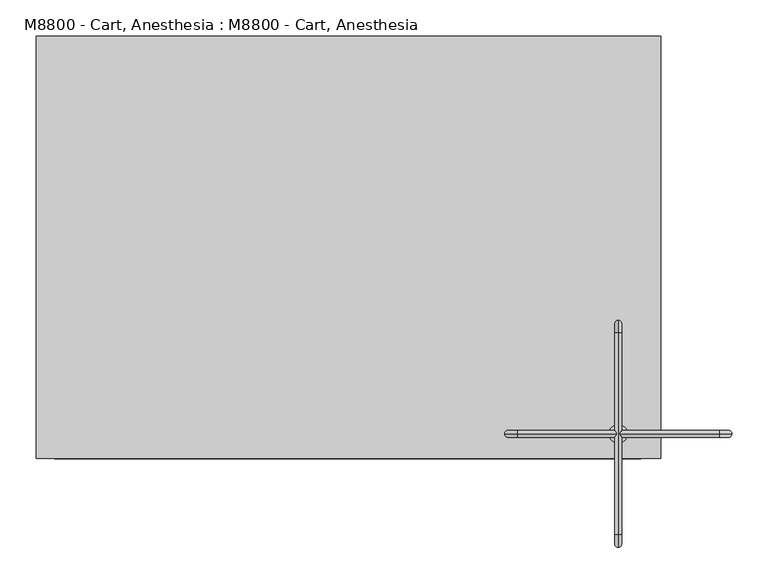
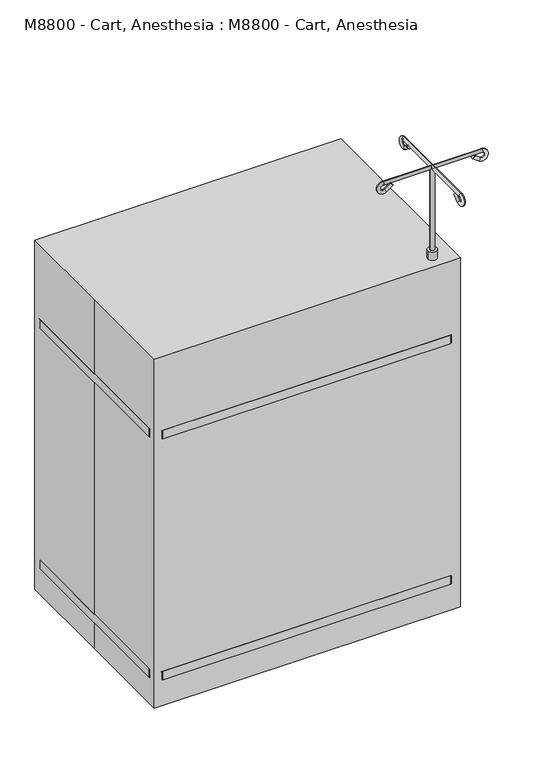
"""IFC4 building model written with IfcOpenShell, lengths in millimetres: proxy geometry, M8800 - Cart, Anesthesia : M8800 - Cart, Anesthesia."""

from ifc_helpers import new_model, si_unit, point, frame, frame_2d, origin, origin_with_axes, place, context, project, spatial, polyline, circle_curve, ellipse_curve, trimmed, segment, composite_curve, outline, extrude, source, transform, mapped, element, save
from ifc_brep_helpers import plane_surface, cylinder_surface, revolved_surface, advanced_brep


def m8800_cart_anesthesia_m8800_cart_anesthesia_5f1830e2(model_context):
    return source(origin(), model_context, "Body", "SolidModel", [
        extrude(outline(composite_curve([segment(trimmed(circle_curve(frame_2d((372.8549743, -257.8577972)), 6.35), [point((366.5049743, -257.8577972))], [point((379.2049743, -257.8577972))], False, "CARTESIAN"), True, "CONTINUOUS"), segment(trimmed(circle_curve(frame_2d((372.8549743, -257.8577972)), 6.35), [point((379.2049743, -257.8577972))], [point((366.5049743, -257.8577972))], False, "CARTESIAN"), True, "CONTINUOUS")], self_intersect=False)), frame((0.0, 0.0, 1066.8), z_axis=(0.0, 0.0, 1.0), x_axis=(1.0, 0.0, 0.0)), (0.0, 0.0, 1.0), 247.65),
        advanced_brep(
        [(372.8549743, -375.3332189, 1305.9580135), (372.8549743, -369.7574508, 1298.2355504), (372.8549743, -387.3355558, 1285.5438178), (372.8549743, -392.9113238, 1293.2662808), (372.8549743, -397.5577972, 1317.1641667), (372.8549743, -397.5577972, 1307.6391667), (372.8549743, -118.1577972, 1317.1641667), (372.8549743, -118.1577972, 1307.6391667), (372.8549743, -128.3800387, 1285.5438178), (372.8549743, -122.8042706, 1293.2662808), (372.8549743, -140.3823755, 1305.9580135), (372.8549743, -145.9581436, 1298.2355504)],
        [
            (0, 1, circle_curve(frame((372.8549743, -372.5453349, 1302.096782), z_axis=(0.0, 0.8107572744902805, 0.5853824748496425), x_axis=(0.0, 0.5853824748496425, -0.8107572744902805)), 4.7625)),
            (1, 0, circle_curve(frame((372.8549743, -372.5453349, 1302.096782), z_axis=(0.0, 0.8107572744902805, 0.5853824748496425), x_axis=(0.0, 0.5853824748496425, -0.8107572744902805)), 4.7625)),
            (1, 2),
            (2, 3, circle_curve(frame((372.8549743, -390.1234398, 1289.4050493), z_axis=(0.0, 0.8107572744902805, 0.5853824748496425), x_axis=(0.0, 0.5853824748496425, -0.8107572744902805)), 4.7625)),
            (3, 0),
            (3, 2, circle_curve(frame((372.8549743, -390.1234398, 1289.4050493), z_axis=(0.0, 0.8107572744902805, 0.5853824748496425), x_axis=(0.0, 0.5853824748496425, -0.8107572744902805)), 4.7625)),
            (4, 5, circle_curve(frame((372.8549743, -397.5577972, 1312.4016667), z_axis=(0.0, -1.0, 0.0), x_axis=(0.0, 0.0, 1.0)), 4.7625)),
            (5, 3, circle_curve(frame((372.8549743, -397.5577972, 1299.7016667), z_axis=(1.0, 0.0, 0.0), x_axis=(0.0, 0.5853824748496496, -0.8107572744902752)), 7.9375)),
            (2, 4, circle_curve(frame((372.8549743, -397.5577972, 1299.7016667), z_axis=(-1.0, 0.0, 0.0), x_axis=(0.0, 0.5853824748496496, -0.8107572744902752)), 17.4625)),
            (5, 4, circle_curve(frame((372.8549743, -397.5577972, 1312.4016667), z_axis=(0.0, -1.0, 0.0), x_axis=(0.0, 0.0, 1.0)), 4.7625)),
            (4, 6),
            (6, 7, circle_curve(frame((372.8549743, -118.1577972, 1312.4016667), z_axis=(0.0, -1.0, 0.0), x_axis=(0.0, 0.0, 1.0)), 4.7625)),
            (7, 5),
            (7, 6, circle_curve(frame((372.8549743, -118.1577972, 1312.4016667), z_axis=(0.0, -1.0, 0.0), x_axis=(0.0, 0.0, 1.0)), 4.7625)),
            (8, 9, circle_curve(frame((372.8549743, -125.5921547, 1289.4050493), z_axis=(0.0, 0.8107572744895717, -0.5853824748506239), x_axis=(0.0, -0.5853824748506239, -0.8107572744895717)), 4.7625)),
            (9, 7, circle_curve(frame((372.8549743, -118.1577972, 1299.7016667), z_axis=(1.0, 0.0, 0.0), x_axis=(0.0, 0.0, 1.0)), 7.9375)),
            (6, 8, circle_curve(frame((372.8549743, -118.1577972, 1299.7016667), z_axis=(-1.0, 0.0, 0.0), x_axis=(0.0, 0.0, 1.0)), 17.4625)),
            (9, 8, circle_curve(frame((372.8549743, -125.5921547, 1289.4050493), z_axis=(0.0, 0.8107572744906105, -0.585382474849185), x_axis=(0.0, -0.585382474849185, -0.8107572744906105)), 4.7625)),
            (10, 11, circle_curve(frame((372.8549743, -143.1702596, 1302.096782), z_axis=(0.0, -0.8107572744898957, 0.5853824748501752), x_axis=(0.0, -0.5853824748501752, -0.8107572744898957)), 4.7625)),
            (11, 10, circle_curve(frame((372.8549743, -143.1702596, 1302.096782), z_axis=(0.0, -0.8107572744898957, 0.5853824748501752), x_axis=(0.0, -0.5853824748501752, -0.8107572744898957)), 4.7625)),
            (8, 11),
            (10, 9),
        ],
        [
            plane_surface(frame((639.5549743, -372.5453349, 1302.096782), z_axis=(0.0, 0.8107572744902805, 0.5853824748496425), x_axis=(-1.0, 0.0, 0.0))),
            cylinder_surface(frame((372.8549743, -372.5453349, 1302.096782), z_axis=(0.0, 0.8107572744902805, 0.5853824748496425), x_axis=(0.0, 0.5853824748496425, -0.8107572744902805)), 4.7625),
            revolved_surface(trimmed(ellipse_curve(frame((372.8549743, -390.1234398, 1289.4050493), z_axis=(0.0, -0.8107572744902751, -0.5853824748496497), x_axis=(0.0, 0.5853824748496497, -0.8107572744902751)), 4.7625, 4.7625), [point((372.8549743, -392.9113238, 1293.2662808))], [point((372.8549743, -387.3355558, 1285.5438178))], True, "CARTESIAN"), (639.5549743, -397.5577972, 1299.7016667), (1.0, 0.0, 0.0)),
            revolved_surface(trimmed(ellipse_curve(frame((372.8549743, -390.1234398, 1289.4050493), z_axis=(0.0, -0.8107572744902751, -0.5853824748496497), x_axis=(0.0, 0.5853824748496497, -0.8107572744902751)), 4.7625, 4.7625), [point((372.8549743, -387.3355558, 1285.5438178))], [point((372.8549743, -392.9113238, 1293.2662808))], True, "CARTESIAN"), (639.5549743, -397.5577972, 1299.7016667), (1.0, 0.0, 0.0)),
            cylinder_surface(frame((372.8549743, -397.5577972, 1312.4016667), z_axis=(0.0, -1.0, 0.0), x_axis=(0.0, 0.0, 1.0)), 4.7625),
            revolved_surface(trimmed(ellipse_curve(frame((372.8549743, -118.1577972, 1312.4016667), z_axis=(0.0, 1.0, 0.0), x_axis=(0.0, 0.0, 1.0)), 4.7625, 4.7625), [point((372.8549743, -118.1577972, 1307.6391667))], [point((372.8549743, -118.1577972, 1317.1641667))], True, "CARTESIAN"), (639.5549743, -118.1577972, 1299.7016667), (1.0, 0.0, 0.0)),
            revolved_surface(trimmed(ellipse_curve(frame((372.8549743, -118.1577972, 1312.4016667), z_axis=(0.0, 1.0, 0.0), x_axis=(0.0, 0.0, 1.0)), 4.7625, 4.7625), [point((372.8549743, -118.1577972, 1317.1641667))], [point((372.8549743, -118.1577972, 1307.6391667))], True, "CARTESIAN"), (639.5549743, -118.1577972, 1299.7016667), (1.0, 0.0, 0.0)),
            plane_surface(frame((639.5549743, -143.1702596, 1302.096782), z_axis=(0.0, -0.8107572744898955, 0.5853824748501754), x_axis=(-1.0, 0.0, 0.0))),
            cylinder_surface(frame((372.8549743, -125.5921547, 1289.4050493), z_axis=(0.0, 0.8107572744898957, -0.5853824748501752), x_axis=(0.0, -0.5853824748501752, -0.8107572744898957)), 4.7625),
        ],
        [
            (0, [[1, 2]]),
            (1, [[3, 4, 5, -2]]),
            (1, [[-5, 6, -3, -1]]),
            (2, [[7, 8, -4, 9]]),
            (3, [[10, -9, -6, -8]]),
            (4, [[11, 12, 13, -7]]),
            (4, [[-13, 14, -11, -10]]),
            (5, [[15, 16, -12, 17]]),
            (6, [[18, -17, -14, -16]]),
            (7, [[19, 20]]),
            (8, [[21, -19, 22, -15]]),
            (8, [[-22, -20, -21, -18]]),
        ],
    ),
        advanced_brep(
        [(255.3795526, -257.8577972, 1305.9580135), (260.9553207, -257.8577972, 1298.2355504), (243.3772158, -257.8577972, 1285.5438178), (237.8014477, -257.8577972, 1293.2662808), (233.1549743, -257.8577972, 1317.1641667), (233.1549743, -257.8577972, 1307.6391667), (512.5549743, -257.8577972, 1317.1641667), (512.5549743, -257.8577972, 1307.6391667), (502.3327328, -257.8577972, 1285.5438178), (507.9085009, -257.8577972, 1293.2662808), (490.330396, -257.8577972, 1305.9580135), (484.7546279, -257.8577972, 1298.2355504)],
        [
            (0, 1, circle_curve(frame((258.1674367, -257.8577972, 1302.096782), z_axis=(0.810757274490287, 0.0, 0.5853824748496332), x_axis=(0.5853824748496332, 0.0, -0.810757274490287)), 4.7625)),
            (1, 0, circle_curve(frame((258.1674367, -257.8577972, 1302.096782), z_axis=(0.810757274490287, 0.0, 0.5853824748496332), x_axis=(0.5853824748496332, 0.0, -0.810757274490287)), 4.7625)),
            (1, 2),
            (2, 3, circle_curve(frame((240.5893317, -257.8577972, 1289.4050493), z_axis=(0.810757274490287, 0.0, 0.5853824748496332), x_axis=(0.5853824748496332, 0.0, -0.810757274490287)), 4.7625)),
            (3, 0),
            (3, 2, circle_curve(frame((240.5893317, -257.8577972, 1289.4050493), z_axis=(0.810757274490287, 0.0, 0.5853824748496332), x_axis=(0.5853824748496332, 0.0, -0.810757274490287)), 4.7625)),
            (4, 5, circle_curve(frame((233.1549743, -257.8577972, 1312.4016667), z_axis=(-1.0, 0.0, 0.0), x_axis=(0.0, 0.0, 1.0)), 4.7625)),
            (5, 3, circle_curve(frame((233.1549743, -257.8577972, 1299.7016667), z_axis=(0.0, -1.0, 0.0), x_axis=(0.5853824748496301, 0.0, -0.8107572744902892)), 7.9375)),
            (2, 4, circle_curve(frame((233.1549743, -257.8577972, 1299.7016667), z_axis=(0.0, 1.0, 0.0), x_axis=(0.5853824748496301, 0.0, -0.8107572744902892)), 17.4625)),
            (5, 4, circle_curve(frame((233.1549743, -257.8577972, 1312.4016667), z_axis=(-1.0, 0.0, 0.0), x_axis=(0.0, 0.0, 1.0)), 4.7625)),
            (4, 6),
            (6, 7, circle_curve(frame((512.5549743, -257.8577972, 1312.4016667), z_axis=(-1.0, 0.0, 0.0), x_axis=(0.0, 0.0, 1.0)), 4.7625)),
            (7, 5),
            (7, 6, circle_curve(frame((512.5549743, -257.8577972, 1312.4016667), z_axis=(-1.0, 0.0, 0.0), x_axis=(0.0, 0.0, 1.0)), 4.7625)),
            (8, 9, circle_curve(frame((505.1206169, -257.8577972, 1289.4050493), z_axis=(0.8107572744899113, 0.0, -0.5853824748501535), x_axis=(-0.5853824748501535, 0.0, -0.8107572744899113)), 4.7625)),
            (9, 7, circle_curve(frame((512.5549743, -257.8577972, 1299.7016667), z_axis=(0.0, -1.0, 0.0), x_axis=(0.0, 0.0, 1.0)), 7.9375)),
            (6, 8, circle_curve(frame((512.5549743, -257.8577972, 1299.7016667), z_axis=(0.0, 1.0, 0.0), x_axis=(0.0, 0.0, 1.0)), 17.4625)),
            (9, 8, circle_curve(frame((505.1206169, -257.8577972, 1289.4050493), z_axis=(0.8107572744899163, 0.0, -0.5853824748501466), x_axis=(-0.5853824748501466, 0.0, -0.8107572744899163)), 4.7625)),
            (10, 11, circle_curve(frame((487.5425119, -257.8577972, 1302.096782), z_axis=(-0.8107572744899004, 0.0, 0.5853824748501685), x_axis=(-0.5853824748501685, 0.0, -0.8107572744899004)), 4.7625)),
            (11, 10, circle_curve(frame((487.5425119, -257.8577972, 1302.096782), z_axis=(-0.8107572744899004, 0.0, 0.5853824748501685), x_axis=(-0.5853824748501685, 0.0, -0.8107572744899004)), 4.7625)),
            (8, 11),
            (10, 9),
        ],
        [
            plane_surface(frame((258.1674367, -473.7577972, 1302.096782), z_axis=(0.810757274490287, 0.0, 0.5853824748496332), x_axis=(0.0, 1.0, 0.0))),
            cylinder_surface(frame((258.1674367, -257.8577972, 1302.096782), z_axis=(0.810757274490287, 0.0, 0.5853824748496332), x_axis=(0.5853824748496332, 0.0, -0.810757274490287)), 4.7625),
            revolved_surface(trimmed(ellipse_curve(frame((240.5893317, -257.8577972, 1289.4050493), z_axis=(-0.8107572744902892, 0.0, -0.5853824748496301), x_axis=(0.5853824748496301, 0.0, -0.8107572744902892)), 4.7625, 4.7625), [point((237.8014477, -257.8577972, 1293.2662808))], [point((243.3772158, -257.8577972, 1285.5438178))], True, "CARTESIAN"), (233.1549743, -473.7577972, 1299.7016667), (0.0, -1.0, 0.0)),
            revolved_surface(trimmed(ellipse_curve(frame((240.5893317, -257.8577972, 1289.4050493), z_axis=(-0.8107572744902892, 0.0, -0.5853824748496301), x_axis=(0.5853824748496301, 0.0, -0.8107572744902892)), 4.7625, 4.7625), [point((243.3772158, -257.8577972, 1285.5438178))], [point((237.8014477, -257.8577972, 1293.2662808))], True, "CARTESIAN"), (233.1549743, -473.7577972, 1299.7016667), (0.0, -1.0, 0.0)),
            cylinder_surface(frame((233.1549743, -257.8577972, 1312.4016667), z_axis=(-1.0, 0.0, 0.0), x_axis=(0.0, 0.0, 1.0)), 4.7625),
            revolved_surface(trimmed(ellipse_curve(frame((512.5549743, -257.8577972, 1312.4016667), z_axis=(1.0, 0.0, 0.0), x_axis=(0.0, 0.0, 1.0)), 4.7625, 4.7625), [point((512.5549743, -257.8577972, 1307.6391667))], [point((512.5549743, -257.8577972, 1317.1641667))], True, "CARTESIAN"), (512.5549743, -473.7577972, 1299.7016667), (0.0, -1.0, 0.0)),
            revolved_surface(trimmed(ellipse_curve(frame((512.5549743, -257.8577972, 1312.4016667), z_axis=(1.0, 0.0, 0.0), x_axis=(0.0, 0.0, 1.0)), 4.7625, 4.7625), [point((512.5549743, -257.8577972, 1317.1641667))], [point((512.5549743, -257.8577972, 1307.6391667))], True, "CARTESIAN"), (512.5549743, -473.7577972, 1299.7016667), (0.0, -1.0, 0.0)),
            plane_surface(frame((487.5425119, -473.7577972, 1302.096782), z_axis=(-0.8107572744899004, 0.0, 0.5853824748501685), x_axis=(0.0, 1.0, 0.0))),
            cylinder_surface(frame((505.1206169, -257.8577972, 1289.4050493), z_axis=(0.8107572744899004, 0.0, -0.5853824748501685), x_axis=(-0.5853824748501685, 0.0, -0.8107572744899004)), 4.7625),
        ],
        [
            (0, [[1, 2]]),
            (1, [[3, 4, 5, -2]]),
            (1, [[-5, 6, -3, -1]]),
            (2, [[7, 8, -4, 9]]),
            (3, [[10, -9, -6, -8]]),
            (4, [[11, 12, 13, -7]]),
            (4, [[-13, 14, -11, -10]]),
            (5, [[15, 16, -12, 17]]),
            (6, [[18, -17, -14, -16]]),
            (7, [[19, 20]]),
            (8, [[21, -19, 22, -15]]),
            (8, [[-22, -20, -21, -18]]),
        ],
    ),
        extrude(outline(polyline([(820.0646026, -374.65), (966.1146026, -374.65), (966.1146026, 120.65), (820.0646026, 120.65), (820.0646026, 127.0), (972.4646026, 127.0), (972.4646026, -381.0), (820.0646026, -381.0), (820.0646026, -374.65)])), frame((0.0, -257.8577972, 0.0), z_axis=(0.0, 1.0, 0.0), x_axis=(0.0, 0.0, 1.0)), (0.0, 0.0, 1.0), 25.4),
        extrude(outline(composite_curve([segment(polyline([(404.3351605, -292.1), (-406.4, -292.1)]), True, "CONTINUOUS"), segment(trimmed(circle_curve(frame_2d((-406.4, -266.7)), 25.4), [point((-406.4, -292.1))], [point((-431.8, -266.7))], False, "CARTESIAN"), True, "CONTINUOUS"), segment(polyline([(-431.8, -266.7), (-431.8, 266.9423102)]), True, "CONTINUOUS"), segment(trimmed(circle_curve(frame_2d((-406.4, 266.9423102)), 25.4), [point((-431.8, 266.9423102))], [point((-406.4, 292.3423102))], False, "CARTESIAN"), True, "CONTINUOUS"), segment(polyline([(-406.4, 292.3423102), (404.3351605, 292.3423102)]), True, "CONTINUOUS"), segment(trimmed(circle_curve(frame_2d((404.3351605, 266.9423102)), 25.4), [point((404.3351605, 292.3423102))], [point((429.7351605, 266.9423102))], False, "CARTESIAN"), True, "CONTINUOUS"), segment(polyline([(429.7351605, 266.9423102), (429.7351605, -266.7)]), True, "CONTINUOUS"), segment(trimmed(circle_curve(frame_2d((404.3351605, -266.7)), 25.4), [point((429.7351605, -266.7))], [point((404.3351605, -292.1))], False, "CARTESIAN"), True, "CONTINUOUS")], self_intersect=False)), frame((0.0, 0.0, 794.6646026), z_axis=(0.0, 0.0, 1.0), x_axis=(1.0, 0.0, 0.0)), (0.0, 0.0, 1.0), 25.4),
        extrude(outline(polyline([(-387.35, -260.35), (-387.35, -241.3), (387.35, -241.3), (387.35, -260.35), (-387.35, -260.35)])), frame((0.0, 0.0, 101.6), z_axis=(0.0, 0.0, 1.0), x_axis=(1.0, 0.0, 0.0)), (0.0, 0.0, 1.0), 693.0646026),
        extrude(outline(polyline([(406.4, -260.35), (387.35, -260.35), (387.35, 247.65), (406.4, 247.65), (406.4, -260.35)])), frame((0.0, 0.0, 101.6), z_axis=(0.0, 0.0, 1.0), x_axis=(1.0, 0.0, 0.0)), (0.0, 0.0, 1.0), 693.0646026),
        extrude(outline(polyline([(-387.35, -260.35), (-406.4, -260.35), (-406.4, 247.65), (-387.35, 247.65), (-387.35, -260.35)])), frame((0.0, 0.0, 101.6), z_axis=(0.0, 0.0, 1.0), x_axis=(1.0, 0.0, 0.0)), (0.0, 0.0, 1.0), 693.0646026),
        extrude(outline(polyline([(-228.6, 31.75), (-236.4377343, 76.2), (-208.0622657, 76.2), (-215.9, 31.75), (-228.6, 31.75)])), frame((-374.65, 0.0, 0.0), z_axis=(1.0, 0.0, 0.0), x_axis=(0.0, 1.0, 0.0)), (0.0, 0.0, 1.0), 3.175),
        extrude(outline(polyline([(-228.6, 31.75), (-236.4377343, 76.2), (-208.0622657, 76.2), (-215.9, 31.75), (-228.6, 31.75)])), frame((-390.525, 0.0, 0.0), z_axis=(1.0, 0.0, 0.0), x_axis=(0.0, 1.0, 0.0)), (0.0, 0.0, 1.0), 3.175),
        extrude(outline(composite_curve([segment(trimmed(circle_curve(frame_2d((-222.25, 31.75)), 31.75), [point((-254.0, 31.75))], [point((-190.5, 31.75))], False, "CARTESIAN"), True, "CONTINUOUS"), segment(trimmed(circle_curve(frame_2d((-222.25, 31.75)), 31.75), [point((-190.5, 31.75))], [point((-254.0, 31.75))], False, "CARTESIAN"), True, "CONTINUOUS")], self_intersect=False)), frame((-387.35, 0.0, 0.0), z_axis=(1.0, 0.0, 0.0), x_axis=(0.0, 1.0, 0.0)), (0.0, 0.0, 1.0), 12.7),
        extrude(outline(polyline([(-228.6, 31.75), (-236.4377343, 76.2), (-208.0622657, 76.2), (-215.9, 31.75), (-228.6, 31.75)])), frame((365.125, 0.0, 0.0), z_axis=(1.0, 0.0, 0.0), x_axis=(0.0, 1.0, 0.0)), (0.0, 0.0, 1.0), 3.175),
        extrude(outline(polyline([(-228.6, 31.75), (-236.4377343, 76.2), (-208.0622657, 76.2), (-215.9, 31.75), (-228.6, 31.75)])), frame((381.0, 0.0, 0.0), z_axis=(1.0, 0.0, 0.0), x_axis=(0.0, 1.0, 0.0)), (0.0, 0.0, 1.0), 3.175),
        extrude(outline(composite_curve([segment(trimmed(circle_curve(frame_2d((-222.25, 31.75)), 31.75), [point((-254.0, 31.75))], [point((-190.5, 31.75))], False, "CARTESIAN"), True, "CONTINUOUS"), segment(trimmed(circle_curve(frame_2d((-222.25, 31.75)), 31.75), [point((-190.5, 31.75))], [point((-254.0, 31.75))], False, "CARTESIAN"), True, "CONTINUOUS")], self_intersect=False)), frame((368.3, 0.0, 0.0), z_axis=(1.0, 0.0, 0.0), x_axis=(0.0, 1.0, 0.0)), (0.0, 0.0, 1.0), 12.7),
        extrude(outline(composite_curve([segment(trimmed(circle_curve(frame_2d((0.0, 158.75)), 127.0), [point((76.2, 260.35))], [point((-76.2, 260.35))], True, "CARTESIAN"), True, "CONTINUOUS"), segment(polyline([(-76.2, 260.35), (-86.3693377, 260.35)]), True, "CONTINUOUS"), segment(trimmed(circle_curve(frame_2d((0.0, 158.75)), 133.35), [point((-86.3693377, 260.35))], [point((86.3693377, 260.35))], False, "CARTESIAN"), True, "CONTINUOUS"), segment(polyline([(86.3693377, 260.35), (76.2, 260.35)]), True, "CONTINUOUS")], self_intersect=False)), frame((0.0, 0.0, 736.6), z_axis=(0.0, 0.0, 1.0), x_axis=(1.0, 0.0, 0.0)), (0.0, 0.0, 1.0), 12.7),
        extrude(outline(polyline([(406.4, 260.35), (406.4, 247.65), (-406.4, 247.65), (-406.4, 260.35), (406.4, 260.35)])), frame((0.0, 0.0, 692.15), z_axis=(0.0, 0.0, 1.0), x_axis=(1.0, 0.0, 0.0)), (0.0, 0.0, 1.0), 101.6),
        extrude(outline(composite_curve([segment(trimmed(circle_curve(frame_2d((0.0, 158.75)), 127.0), [point((76.2, 260.35))], [point((-76.2, 260.35))], True, "CARTESIAN"), True, "CONTINUOUS"), segment(polyline([(-76.2, 260.35), (-86.3693377, 260.35)]), True, "CONTINUOUS"), segment(trimmed(circle_curve(frame_2d((0.0, 158.75)), 133.35), [point((-86.3693377, 260.35))], [point((86.3693377, 260.35))], False, "CARTESIAN"), True, "CONTINUOUS"), segment(polyline([(86.3693377, 260.35), (76.2, 260.35)]), True, "CONTINUOUS")], self_intersect=False)), frame((0.0, 0.0, 628.65), z_axis=(0.0, 0.0, 1.0), x_axis=(1.0, 0.0, 0.0)), (0.0, 0.0, 1.0), 12.7),
        extrude(outline(polyline([(406.4, 260.35), (406.4, 247.65), (-406.4, 247.65), (-406.4, 260.35), (406.4, 260.35)])), frame((0.0, 0.0, 584.2), z_axis=(0.0, 0.0, 1.0), x_axis=(1.0, 0.0, 0.0)), (0.0, 0.0, 1.0), 101.6),
        extrude(outline(composite_curve([segment(trimmed(circle_curve(frame_2d((0.0, 158.75)), 127.0), [point((76.2, 260.35))], [point((-76.2, 260.35))], True, "CARTESIAN"), True, "CONTINUOUS"), segment(polyline([(-76.2, 260.35), (-86.3693377, 260.35)]), True, "CONTINUOUS"), segment(trimmed(circle_curve(frame_2d((0.0, 158.75)), 133.35), [point((-86.3693377, 260.35))], [point((86.3693377, 260.35))], False, "CARTESIAN"), True, "CONTINUOUS"), segment(polyline([(86.3693377, 260.35), (76.2, 260.35)]), True, "CONTINUOUS")], self_intersect=False)), frame((0.0, 0.0, 342.9), z_axis=(0.0, 0.0, 1.0), x_axis=(1.0, 0.0, 0.0)), (0.0, 0.0, 1.0), 12.7),
        extrude(outline(composite_curve([segment(trimmed(circle_curve(frame_2d((-0.7312252, 158.75)), 127.0), [point((75.4687748, 260.35))], [point((-76.9312252, 260.35))], True, "CARTESIAN"), True, "CONTINUOUS"), segment(polyline([(-76.9312252, 260.35), (-87.1005629, 260.35)]), True, "CONTINUOUS"), segment(trimmed(circle_curve(frame_2d((-0.7312252, 158.75)), 133.35), [point((-87.1005629, 260.35))], [point((85.6381125, 260.35))], False, "CARTESIAN"), True, "CONTINUOUS"), segment(polyline([(85.6381125, 260.35), (75.4687748, 260.35)]), True, "CONTINUOUS")], self_intersect=False)), frame((0.0, 0.0, 488.95), z_axis=(0.0, 0.0, 1.0), x_axis=(1.0, 0.0, 0.0)), (0.0, 0.0, 1.0), 12.7),
        extrude(outline(polyline([(406.4, 260.35), (406.4, 247.65), (-406.4, 247.65), (-406.4, 260.35), (406.4, 260.35)])), frame((0.0, 0.0, 101.6), z_axis=(0.0, 0.0, 1.0), x_axis=(1.0, 0.0, 0.0)), (0.0, 0.0, 1.0), 304.8),
        extrude(outline(polyline([(406.4, 260.35), (406.4, 247.65), (-406.4, 247.65), (-406.4, 260.35), (406.4, 260.35)])), frame((0.0, 0.0, 412.75), z_axis=(0.0, 0.0, 1.0), x_axis=(1.0, 0.0, 0.0)), (0.0, 0.0, 1.0), 165.1),
        extrude(outline(polyline([(247.65, 31.75), (234.95, 31.75), (227.1122657, 76.2), (255.4877343, 76.2), (247.65, 31.75)])), frame((-374.65, 0.0, 0.0), z_axis=(1.0, 0.0, 0.0), x_axis=(0.0, 1.0, 0.0)), (0.0, 0.0, 1.0), 3.175),
        extrude(outline(polyline([(247.65, 31.75), (234.95, 31.75), (227.1122657, 76.2), (255.4877343, 76.2), (247.65, 31.75)])), frame((-390.525, 0.0, 0.0), z_axis=(1.0, 0.0, 0.0), x_axis=(0.0, 1.0, 0.0)), (0.0, 0.0, 1.0), 3.175),
        extrude(outline(composite_curve([segment(trimmed(circle_curve(frame_2d((241.3, 31.75)), 31.75), [point((273.05, 31.75))], [point((209.55, 31.75))], False, "CARTESIAN"), True, "CONTINUOUS"), segment(trimmed(circle_curve(frame_2d((241.3, 31.75)), 31.75), [point((209.55, 31.75))], [point((273.05, 31.75))], False, "CARTESIAN"), True, "CONTINUOUS")], self_intersect=False)), frame((-387.35, 0.0, 0.0), z_axis=(1.0, 0.0, 0.0), x_axis=(0.0, 1.0, 0.0)), (0.0, 0.0, 1.0), 12.7),
        extrude(outline(polyline([(247.65, 31.75), (234.95, 31.75), (227.1122657, 76.2), (255.4877343, 76.2), (247.65, 31.75)])), frame((365.125, 0.0, 0.0), z_axis=(1.0, 0.0, 0.0), x_axis=(0.0, 1.0, 0.0)), (0.0, 0.0, 1.0), 3.175),
        extrude(outline(polyline([(247.65, 31.75), (234.95, 31.75), (227.1122657, 76.2), (255.4877343, 76.2), (247.65, 31.75)])), frame((381.0, 0.0, 0.0), z_axis=(1.0, 0.0, 0.0), x_axis=(0.0, 1.0, 0.0)), (0.0, 0.0, 1.0), 3.175),
        extrude(outline(composite_curve([segment(trimmed(circle_curve(frame_2d((241.3, 31.75)), 31.75), [point((273.05, 31.75))], [point((209.55, 31.75))], False, "CARTESIAN"), True, "CONTINUOUS"), segment(trimmed(circle_curve(frame_2d((241.3, 31.75)), 31.75), [point((209.55, 31.75))], [point((273.05, 31.75))], False, "CARTESIAN"), True, "CONTINUOUS")], self_intersect=False)), frame((368.3, 0.0, 0.0), z_axis=(1.0, 0.0, 0.0), x_axis=(0.0, 1.0, 0.0)), (0.0, 0.0, 1.0), 12.7),
        extrude(outline(composite_curve([segment(trimmed(circle_curve(frame_2d((372.8549743, -257.8577972)), 12.7), [point((360.1549743, -257.8577972))], [point((385.5549743, -257.8577972))], False, "CARTESIAN"), True, "CONTINUOUS"), segment(trimmed(circle_curve(frame_2d((372.8549743, -257.8577972)), 12.7), [point((385.5549743, -257.8577972))], [point((360.1549743, -257.8577972))], False, "CARTESIAN"), True, "CONTINUOUS")], self_intersect=False)), frame((0.0, 0.0, 820.0646026), z_axis=(0.0, 0.0, 1.0), x_axis=(1.0, 0.0, 0.0)), (0.0, 0.0, 1.0), 246.7353974),
        extrude(outline(composite_curve([segment(polyline([(404.3351605, -292.1), (-406.4, -292.1)]), True, "CONTINUOUS"), segment(trimmed(circle_curve(frame_2d((-406.4, -266.7)), 25.4), [point((-406.4, -292.1))], [point((-431.8, -266.7))], False, "CARTESIAN"), True, "CONTINUOUS"), segment(polyline([(-431.8, -266.7), (-431.8, 266.9423102)]), True, "CONTINUOUS"), segment(trimmed(circle_curve(frame_2d((-406.4, 266.9423102)), 25.4), [point((-431.8, 266.9423102))], [point((-406.4, 292.3423102))], False, "CARTESIAN"), True, "CONTINUOUS"), segment(polyline([(-406.4, 292.3423102), (404.3351605, 292.3423102)]), True, "CONTINUOUS"), segment(trimmed(circle_curve(frame_2d((404.3351605, 266.9423102)), 25.4), [point((404.3351605, 292.3423102))], [point((429.7351605, 266.9423102))], False, "CARTESIAN"), True, "CONTINUOUS"), segment(polyline([(429.7351605, 266.9423102), (429.7351605, -266.7)]), True, "CONTINUOUS"), segment(trimmed(circle_curve(frame_2d((404.3351605, -266.7)), 25.4), [point((429.7351605, -266.7))], [point((404.3351605, -292.1))], False, "CARTESIAN"), True, "CONTINUOUS")], self_intersect=False)), frame((0.0, 0.0, 76.2), z_axis=(0.0, 0.0, 1.0), x_axis=(1.0, 0.0, 0.0)), (0.0, 0.0, 1.0), 25.4),
        extrude(outline(polyline([(-431.8, -292.1), (-431.8, 0.0), (-431.8, 292.1), (431.8, 292.1), (431.8, -292.1), (-431.8, -292.1)])), origin_with_axes(), (0.0, 0.0, 1.0), 1041.4),
    ])


if __name__ == "__main__":
    model = new_model("IFC4")
    model_context = context("Model", 3, world=origin())
    ifc_project = project(units=[si_unit("LENGTHUNIT", "METRE", prefix="MILLI")], contexts=[model_context])
    site = spatial("IfcSite", under=ifc_project)
    building = spatial("IfcBuilding", under=site)
    placement = place(None, origin())
    m8800_cart_anesthesia_m8800_cart_anesthesia_shape = m8800_cart_anesthesia_m8800_cart_anesthesia_5f1830e2(model_context)
    element("IfcBuildingElementProxy", 1, Name="M8800 - Cart, Anesthesia : M8800 - Cart, Anesthesia", ObjectType="M8800 - Cart, Anesthesia : M8800 - Cart, Anesthesia", at=placement, inside=building, context=model_context, shape_type="MappedRepresentation", body=[
        mapped(m8800_cart_anesthesia_m8800_cart_anesthesia_shape, transform((0.0, 0.0, 0.0), x_axis=(1.0, 0.0, 0.0), y_axis=(0.0, 1.0, 0.0), z_axis=(0.0, 0.0, 1.0))),
    ])
    save(model, "model.ifc")

# Revit data of these elements
# Type "M8800 - Cart, Anesthesia : M8800 - Cart, Anesthesia"
#   Watts2 = "0"
#   Watts1 = "0"
#   Unit_Issue = "EA"
#   UTIL_6_Misc = "-"
#   UTIL_5_NonMedGas = "-"
#   UTIL_4_MiscGas = "-"
#   UTIL_3_MedGas = "-"
#   UTIL_2_Elec = "-"
#   UTIL_1_WaterDrain = "-"
#   Nomenclature = "Cart, Anesthesia"
#   NSN = "6530"
#   Location [instance default] = ""
#   JSN = "M8800"
#   Fund_Source_VA = "-"
#   Fund_Source_Navy = "-"
#   Fund_Source_Army = "-"
#   Fund_Source_AF = "-"
#   ELEC_Volts2 = "0"
#   ELEC_Volts1 = "0"
#   ELEC_Phase2 = "0"
#   ELEC_Phase1 = "0"
#   ELEC_HertzSwitch = "0"
#   ELEC_HertzDependent = "0"
#   ELEC_Hertz = "0"
#   ELEC_Amps2 = "0"
#   ELEC_Amps1 = "0"
#   DetailDescription = "Mobile anesthesia cart. The cart shall be built of stainless steel and mounted on 4\" casters for easy mobility. It shall be capable of being equipped with bottle holders, adjustable IV pole, storage drawers, shelves and a top bar/rail."
#   CAT_VA = "C"
#   CAT_Navy = "C"
#   CAT_IHS = "-"
#   CAT_Army = "C"
#   CAT_AF = "C"
#   BTUperhour = "0"
#   Weight_IP = 145
#   DIM_Width_IP = 2' - 10"
#   DIM_Height_IP = 3' - 5"
#   DIM_Depth_IP = 1' - 11"
#   finish [instance default] = none
# Element 1 (IfcBuildingElementProxy, "M8800 - Cart, Anesthesia : M8800 - Cart, Anesthesia")
#   Location = "XDCY1"
#   Materials on its faces: "EquipSpace"
# Materials
#   "EquipSpace": class "Unassigned", colour RGB 221 217 195, transparency 0.5
